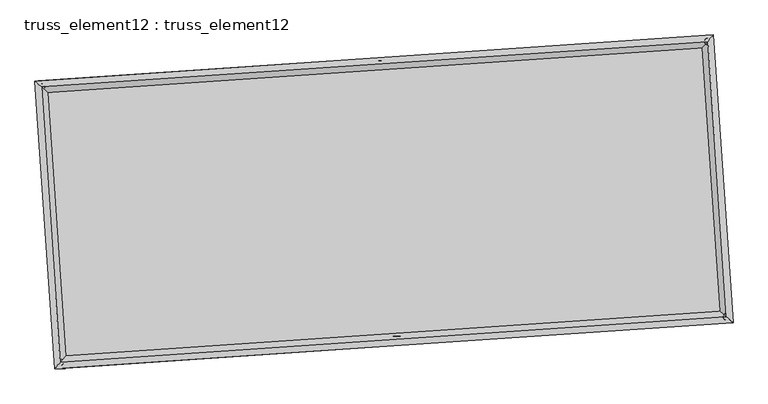
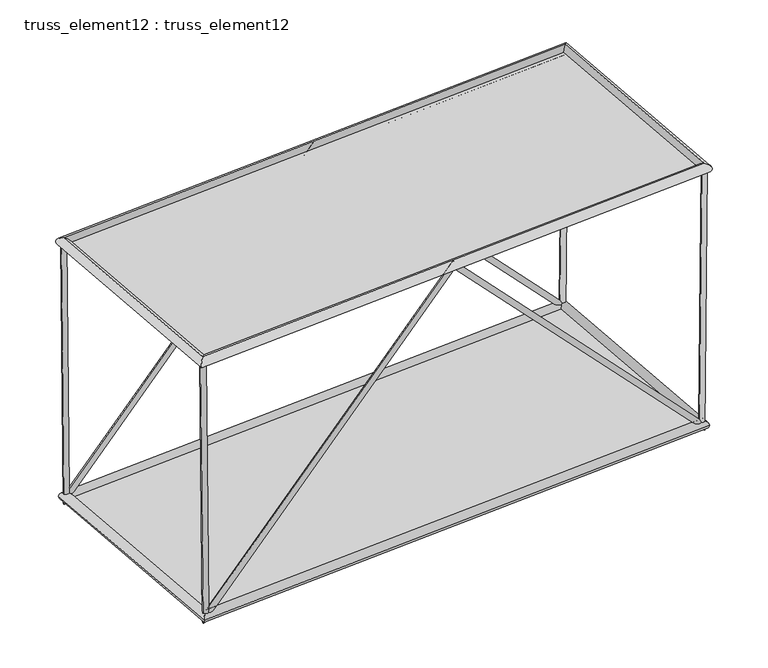
"""IFC4 building model written with IfcOpenShell, lengths in millimetres: plate geometry, truss_element12 : truss_element12."""

import ifcopenshell
import ifcopenshell.guid

model = None  # the IFC model being written
_history = None  # IfcOwnerHistory: only IFC2X3 demands one
_inside = {}  # id of a spatial element -> (the spatial element, [elements in it])
_under = {}  # id of a project, library or spatial element -> (it, [spatial elements below it])
_declared = {}  # id of a project -> (the project, [libraries it declares])
_typed = {}  # id of a type object -> (the type object, [elements of that type])
_made_of = {}  # id of a material, layer set ... -> (it, [elements and type objects made of it])


def new_model(schema):
    """Start an empty IFC model of exactly this schema.

    Asked for "IFC4X3", IfcOpenShell would pick the latest addendum, in which some entities
    have other attributes; the version numbers below select the first issue.
    IFC2X3 requires an IfcOwnerHistory on every rooted entity: one is made here for all.
    """
    global model, _history
    if schema == "IFC4X3":
        model = ifcopenshell.file(schema_version=(4, 3, 0, 0))
    else:
        model = ifcopenshell.file(schema=schema)
    _inside.clear()
    _under.clear()
    _declared.clear()
    _typed.clear()
    _made_of.clear()
    _history = None
    if model.schema == "IFC2X3":
        org = make("IfcOrganization", Name="unknown")
        user = make(
            "IfcPersonAndOrganization",
            ThePerson=make("IfcPerson", FamilyName="unknown"),
            TheOrganization=org,
        )
        app = make(
            "IfcApplication",
            ApplicationDeveloper=org,
            Version="unknown",
            ApplicationFullName="unknown",
            ApplicationIdentifier="unknown",
        )
        _history = make(
            "IfcOwnerHistory",
            OwningUser=user,
            OwningApplication=app,
            ChangeAction="ADDED",
            CreationDate=0,
        )
    return model


def make(cls, **values):
    """One entity of the class cls with the attributes given. An attribute that is None is left unset."""
    return model.create_entity(
        cls, **{name: value for name, value in values.items() if value is not None}
    )


def rooted(cls, **values):
    """An entity with a GlobalId (a new one), such as an element, a storey or a relation."""
    return make(cls, GlobalId=ifcopenshell.guid.new(), OwnerHistory=_history, **values)


def si_unit(unit_type, name, prefix=None):
    """IfcSIUnit, for example si_unit("LENGTHUNIT", "METRE", prefix="MILLI")."""
    return make("IfcSIUnit", UnitType=unit_type, Prefix=prefix, Name=name)


def assignment(units):
    """IfcUnitAssignment: the units of a project."""
    return None if units is None else make("IfcUnitAssignment", Units=units)


def point(xyz):
    """IfcCartesianPoint."""
    return None if xyz is None else make("IfcCartesianPoint", Coordinates=xyz)


def direction(xyz):
    """IfcDirection."""
    return None if xyz is None else make("IfcDirection", DirectionRatios=xyz)


def frame(location, z_axis=None, x_axis=None):
    """IfcAxis2Placement3D, a coordinate frame: its origin and axes. An axis left out is left unset."""
    return make(
        "IfcAxis2Placement3D",
        Location=point(location),
        Axis=direction(z_axis),
        RefDirection=direction(x_axis),
    )


def origin():
    """The frame at (0, 0, 0) with its axes left unset."""
    return frame((0.0, 0.0, 0.0))


def origin_with_axes():
    """The frame at (0, 0, 0) with the z axis (0, 0, 1) and the x axis (1, 0, 0) written out."""
    return frame((0.0, 0.0, 0.0), z_axis=(0.0, 0.0, 1.0), x_axis=(1.0, 0.0, 0.0))


def place(relative_to, where):
    """IfcLocalPlacement: puts the frame where relative to a parent placement (None: the world)."""
    return make(
        "IfcLocalPlacement", PlacementRelTo=relative_to, RelativePlacement=where
    )


def context(
    kind, dimensions, precision=None, world=None, true_north=None, identifier=None
):
    """IfcGeometricRepresentationContext, for example the 3D "Model" context."""
    return make(
        "IfcGeometricRepresentationContext",
        ContextIdentifier=identifier,
        ContextType=kind,
        CoordinateSpaceDimension=dimensions,
        Precision=precision,
        WorldCoordinateSystem=world,
        TrueNorth=true_north,
    )


def project(units=None, contexts=None):
    """IfcProject with its units and contexts."""
    return rooted(
        "IfcProject",
        Name="project",
        RepresentationContexts=contexts,
        UnitsInContext=assignment(units),
    )


def spatial(cls, under=None, at=None, **own):
    """A site, building, storey or space (cls), placed at a placement, below another one or the project."""
    s = rooted(cls, ObjectPlacement=at, **own)
    if under is not None:
        _under.setdefault(under.id(), (under, []))[1].append(s)
    return s


def polyline(points):
    """IfcPolyline through the points."""
    return make("IfcPolyline", Points=[point(p) for p in points])


def circle_curve(where, radius):
    """IfcCircle in the frame where."""
    return make("IfcCircle", Position=where, Radius=radius)


def ellipse_curve(where, semi_axis1, semi_axis2):
    """IfcEllipse in the frame where."""
    return make(
        "IfcEllipse", Position=where, SemiAxis1=semi_axis1, SemiAxis2=semi_axis2
    )


def outline(outer, holes=None, kind="AREA"):
    """IfcArbitraryClosedProfileDef: a profile drawn as a closed curve; with holes, ...WithVoids."""
    if holes is None:
        return make("IfcArbitraryClosedProfileDef", ProfileType=kind, OuterCurve=outer)
    return make(
        "IfcArbitraryProfileDefWithVoids",
        ProfileType=kind,
        OuterCurve=outer,
        InnerCurves=holes,
    )


def extrude(swept, where, along, depth):
    """IfcExtrudedAreaSolid: the profile swept, set in the frame where, extruded along a direction by depth."""
    return make(
        "IfcExtrudedAreaSolid",
        SweptArea=swept,
        Position=where,
        ExtrudedDirection=direction(along),
        Depth=depth,
    )


def shape(context_of_items, identifier, shape_type, items):
    """IfcShapeRepresentation: the items that make up one representation, for example the "Body"."""
    return make(
        "IfcShapeRepresentation",
        ContextOfItems=context_of_items,
        RepresentationIdentifier=identifier,
        RepresentationType=shape_type,
        Items=items,
    )


def source(mapping_origin, context_of_items, identifier, shape_type, items):
    """IfcRepresentationMap: a shape defined once, which mapped items show again and again."""
    return make(
        "IfcRepresentationMap",
        MappingOrigin=mapping_origin,
        MappedRepresentation=shape(context_of_items, identifier, shape_type, items),
    )


def transform(
    local_origin,
    x_axis=None,
    y_axis=None,
    z_axis=None,
    scale=None,
    scale2=None,
    scale3=None,
    uniform=True,
):
    """IfcCartesianTransformationOperator3D, or its non-uniform kind. x_axis, y_axis, z_axis: its Axis1, 2, 3."""
    if uniform:
        return make(
            "IfcCartesianTransformationOperator3D",
            Axis1=direction(x_axis),
            Axis2=direction(y_axis),
            LocalOrigin=point(local_origin),
            Scale=scale,
            Axis3=direction(z_axis),
        )
    return make(
        "IfcCartesianTransformationOperator3DnonUniform",
        Axis1=direction(x_axis),
        Axis2=direction(y_axis),
        LocalOrigin=point(local_origin),
        Scale=scale,
        Axis3=direction(z_axis),
        Scale2=scale2,
        Scale3=scale3,
    )


def mapped(mapping_source, mapping_target):
    """IfcMappedItem: shows the shape of a source again, moved by a transform."""
    return make(
        "IfcMappedItem", MappingSource=mapping_source, MappingTarget=mapping_target
    )


def made_of(thing, what):
    """Note that an element or type object is made of a material, layer set ...; save() writes the relation."""
    if what is not None:
        _made_of.setdefault(what.id(), (what, []))[1].append(thing)
    return thing


def element(
    cls,
    number,
    at=None,
    inside=None,
    cuts=None,
    type_object=None,
    material=None,
    context=None,
    identifier="Body",
    shape_type=None,
    held_by="IfcProductDefinitionShape",
    body=None,
    shapes=None,
    **own,
):
    """One element of the class cls, such as IfcWall. Its Tag is "e" and its number.

    at: its placement. inside: the storey or other place that contains it. cuts: it is an
    opening in that element (IfcRelVoidsElement). A single representation is given by context,
    identifier, shape_type and body (its items); several are given by shapes. held_by: the class
    of the entity that holds the representations. save() writes the other relations.
    """
    e = rooted(cls, Tag="e%d" % number, ObjectPlacement=at, **own)
    if body is not None:
        shapes = [shape(context, identifier, shape_type, body)]
    if shapes is not None:
        e.Representation = make(held_by, Representations=shapes)
    if inside is not None:
        _inside.setdefault(inside.id(), (inside, []))[1].append(e)
    if cuts is not None:
        rooted(
            "IfcRelVoidsElement", RelatingBuildingElement=cuts, RelatedOpeningElement=e
        )
    if type_object is not None:
        _typed.setdefault(type_object.id(), (type_object, []))[1].append(e)
    return made_of(e, material)


def aggregate(whole, parts):
    """IfcRelAggregates: a whole, such as a stair, and the parts it consists of."""
    return rooted("IfcRelAggregates", RelatingObject=whole, RelatedObjects=parts)


def save(model, path):
    """Write the relations noted so far, then the file.

    IfcRelAggregates (storeys below a building ...), IfcRelContainedInSpatialStructure (elements
    in a storey), IfcRelDefinesByType, IfcRelAssociatesMaterial and IfcRelDeclares: one each for
    every whole, place, type object, material and project.
    """
    for whole, parts in _under.values():
        aggregate(whole, parts)
    for where, things in _inside.values():
        rooted(
            "IfcRelContainedInSpatialStructure",
            RelatedElements=things,
            RelatingStructure=where,
        )
    for kind, things in _typed.values():
        rooted("IfcRelDefinesByType", RelatedObjects=things, RelatingType=kind)
    for what, things in _made_of.values():
        rooted("IfcRelAssociatesMaterial", RelatedObjects=things, RelatingMaterial=what)
    for by, libraries in _declared.values():
        rooted("IfcRelDeclares", RelatingContext=by, RelatedDefinitions=libraries)
    model.write(path)


def plane_surface(at):
    """IfcPlane: the flat surface through the origin of the frame at, square to its z axis."""
    return make("IfcPlane", Position=at)


def cylinder_surface(at, radius):
    """IfcCylindricalSurface: all points at the distance radius from the z axis of the frame at."""
    return make("IfcCylindricalSurface", Position=at, Radius=radius)


def advanced_brep(points, edges, surfaces, faces):
    """IfcAdvancedBrep: a solid bounded by faces that lie on surfaces and meet in shared edges.

    An edge is (start, end): straight between two places in points (the first is 0);
    or (start, end, curve); or (start, end, curve, False) where it runs against its curve.
    A face is (place in surfaces, loops), or (place, loops, False) where it looks against
    its surface's normal. A loop lists edges by number (the first is 1), with a minus sign
    where the edge is run from its end to its start. The first loop is the outer one.
    """
    corners = [point(p) for p in points]
    vertices = [make("IfcVertexPoint", VertexGeometry=c) for c in corners]
    made = []
    for start, end, *more in edges:
        made.append(
            make(
                "IfcEdgeCurve",
                EdgeStart=vertices[start],
                EdgeEnd=vertices[end],
                EdgeGeometry=more[0] if more else make("IfcPolyline", Points=[corners[start], corners[end]]),
                SameSense=more[1] if len(more) > 1 else True,
            )
        )
    hull = []
    for where, loops, *sense in faces:
        bounds = []
        for j, loop in enumerate(loops):
            ring = [make("IfcOrientedEdge", EdgeElement=made[abs(k) - 1], Orientation=k > 0) for k in loop]
            bounds.append(
                make(
                    "IfcFaceOuterBound" if j == 0 else "IfcFaceBound",
                    Bound=make("IfcEdgeLoop", EdgeList=ring),
                    Orientation=True,
                )
            )
        hull.append(make("IfcAdvancedFace", Bounds=bounds, FaceSurface=surfaces[where], SameSense=sense[0] if sense else True))
    return make("IfcAdvancedBrep", Outer=make("IfcClosedShell", CfsFaces=hull))


def truss_element12_truss_element12_ac9c6d62(model_context):
    return source(origin(), model_context, "Body", "SolidModel", [
        advanced_brep(
        [(-3716.0930721, 2272.7361645, 5000.2487185), (-3815.1912006, 2259.3752454, 4999.2255971), (-3666.1964298, 2276.1384269, 122.8985351), (-3762.790453, 2262.9482532, -122.8985351), (1063.2705222, 2598.6227999, 5071.8637093), (1063.7254289, 2592.0500239, 4927.6196851), (5793.6135203, 2921.1669073, 122.9048123), (5891.1474567, 2921.2135812, -122.9048123), (5842.6407291, 2924.5098863, 5000.248885), (5942.6354458, 2924.7243515, 4999.2435881)],
        [
            (0, 1, circle_curve(frame((-3765.6421364, 2266.055705, 4999.7371578), z_axis=(-0.010229738989149566, -0.0006975270147916147, 0.9999474315664186), x_axis=(-0.13360930371043286, 0.991033852899563, -0.0006755509311635323)), 50.0)),
            (1, 0, circle_curve(frame((-3765.6421364, 2266.055705, 4999.7371578), z_axis=(-0.010229738989149566, -0.0006975270147916147, 0.9999474315664186), x_axis=(-0.13360930371043286, 0.991033852899563, -0.0006755509311635323)), 50.0)),
            (0, 2),
            (2, 3, ellipse_curve(frame((-3714.4934414, 2269.54334, 0.0), z_axis=(-0.9276876380424472, -0.06325549356725499, 0.36795976513307577), x_axis=(0.367107348096881, 0.02503165456104934, 0.9298417130045371)), 132.4592623, 50.0)),
            (3, 1),
            (3, 2, ellipse_curve(frame((-3714.4934414, 2269.54334, 0.0), z_axis=(-0.9276876380424472, -0.06325549356725499, 0.36795976513307577), x_axis=(0.367107348096881, 0.02503165456104934, 0.9298417130045371)), 132.4592623, 50.0)),
            (2, 4),
            (4, 5, ellipse_curve(frame((1063.4979755, 2595.3364119, 4999.7416972), z_axis=(-0.9976833949926481, -0.0680282381549069, -4.657770887694116e-05), x_axis=(4.6469806773723855e-05, 3.1685994757026087e-06, -0.9999999989152586)), 72.2790583, 50.0)),
            (5, 3),
            (5, 4, ellipse_curve(frame((1063.4979755, 2595.3364119, 4999.7416972), z_axis=(-0.9976833949926481, -0.0680282381549069, -4.657770887694116e-05), x_axis=(4.6469806773723855e-05, 3.1685994757026087e-06, -0.9999999989152586)), 72.2790583, 50.0)),
            (4, 6),
            (6, 7, ellipse_curve(frame((5842.3804885, 2921.1902443, 0.0), z_axis=(-0.9276377400160161, -0.06325209121051292, -0.3680861261382656), x_axis=(-0.3672334163736703, -0.025040250677613285, 0.9297916991157348)), 132.4731533, 50.0)),
            (7, 5),
            (7, 6, ellipse_curve(frame((5842.3804885, 2921.1902443, 0.0), z_axis=(-0.9276377400160161, -0.06325209121051292, -0.3680861261382656), x_axis=(-0.3672334163736703, -0.025040250677613285, 0.9297916991157348)), 132.4731533, 50.0)),
            (8, 9, circle_curve(frame((5892.6380875, 2924.6171189, 4999.7462366), z_axis=(0.010051519791738127, 0.000685374925194703, 0.9999492473176268), x_axis=(-0.0021514333546637375, 0.9999974653609742, -0.0006637817017735374)), 50.0)),
            (9, 8, circle_curve(frame((5892.6380875, 2924.6171189, 4999.7462366), z_axis=(0.010051519791738127, 0.000685374925194703, 0.9999492473176268), x_axis=(-0.0021514333546637375, 0.9999974653609742, -0.0006637817017735374)), 50.0)),
            (6, 8),
            (9, 7),
        ],
        [
            plane_surface(frame((-3765.6421364, 2316.0556928, 4999.772036), z_axis=(-0.01022973898914786, -0.0006975270147901555, 0.9999474315664189), x_axis=(0.9999476748511464, -7.13589268563908e-06, 0.010229736500278365))),
            cylinder_surface(frame((-3765.6421364, 2266.055705, 4999.7371578), z_axis=(-0.010229738989149566, -0.0006975270147916147, 0.9999474315664186), x_axis=(-0.13360930371043286, 0.991033852899563, -0.0006755509311635323)), 50.0),
            cylinder_surface(frame((-3714.4934414, 2269.54334, 0.0), z_axis=(-0.6901272026448979, -0.047057150529254535, -0.722156540338447), x_axis=(-0.02041139550442059, 0.9987523879545969, -0.04557458160589792)), 50.0),
            cylinder_surface(frame((1063.4979755, 2595.3364119, 4999.7416972), z_axis=(-0.6901943166001666, -0.047061726774740395, 0.7220920988390669), x_axis=(-0.11534522502427148, 0.9922792109969094, -0.04557901367352192)), 50.0),
            plane_surface(frame((5892.6380875, 2874.6171306, 4999.7805071), z_axis=(0.010051519791740156, 0.0006853749251952957, 0.9999492473176268), x_axis=(0.9999494821989141, -6.889407663024368e-06, -0.010051517430706975))),
            cylinder_surface(frame((5842.3804885, 2921.1902443, 0.0), z_axis=(-0.010051519791738127, -0.000685374925194703, -0.9999492473176268), x_axis=(-0.0021514333546637375, 0.9999974653609742, -0.0006637817017735374)), 50.0),
        ],
        [
            (0, [[1, 2]]),
            (1, [[-1, 3, 4, 5]]),
            (1, [[-2, -5, 6, -3]]),
            (2, [[-4, 7, 8, 9]]),
            (2, [[-6, -9, 10, -7]]),
            (3, [[-8, 11, 12, 13]]),
            (3, [[-10, -13, 14, -11]]),
            (4, [[15, 16]]),
            (5, [[-12, 17, -16, 18]]),
            (5, [[-14, -18, -15, -17]]),
        ],
    ),
        advanced_brep(
        [(-3443.9801192, -1717.9974198, 5000.2487185), (-3543.0782477, -1731.3583389, 4999.2255971), (-3394.0834769, -1714.5951574, 122.8985351), (-3490.6775001, -1727.7853311, -122.8985351), (1335.3834751, -1392.1107844, 5071.8637093), (1335.8383818, -1398.6835604, 4927.6196851), (6065.7264732, -1069.566677, 122.9048123), (6163.2604096, -1069.5200031, -122.9048123), (6114.753682, -1066.223698, 5000.248885), (6214.7483988, -1066.0092328, 4999.2435881)],
        [
            (0, 1, circle_curve(frame((-3493.5291834, -1724.6778793, 4999.7371578), z_axis=(-0.010229738989149568, -0.0006975270147916012, 0.9999474315664186), x_axis=(-0.1336093037104329, 0.991033852899563, -0.0006755509311635461)), 50.0)),
            (1, 0, circle_curve(frame((-3493.5291834, -1724.6778793, 4999.7371578), z_axis=(-0.010229738989149568, -0.0006975270147916012, 0.9999474315664186), x_axis=(-0.1336093037104329, 0.991033852899563, -0.0006755509311635461)), 50.0)),
            (0, 2),
            (2, 3, ellipse_curve(frame((-3442.3804885, -1721.1902443, 0.0), z_axis=(-0.9276876380424474, -0.06325549356725498, 0.3679597651330757), x_axis=(0.3671073480968811, 0.025031654561049346, 0.9298417130045371)), 132.4592623, 50.0)),
            (3, 1),
            (3, 2, ellipse_curve(frame((-3442.3804885, -1721.1902443, 0.0), z_axis=(-0.9276876380424474, -0.06325549356725498, 0.3679597651330757), x_axis=(0.3671073480968811, 0.025031654561049346, 0.9298417130045371)), 132.4592623, 50.0)),
            (2, 4),
            (4, 5, ellipse_curve(frame((1335.6109285, -1395.3971724, 4999.7416972), z_axis=(-0.9976833949926481, -0.06802823815490679, -4.657770887694117e-05), x_axis=(4.6469806773723855e-05, 3.1685994756065187e-06, -0.9999999989152586)), 72.2790583, 50.0)),
            (5, 3),
            (5, 4, ellipse_curve(frame((1335.6109285, -1395.3971724, 4999.7416972), z_axis=(-0.9976833949926481, -0.06802823815490679, -4.657770887694117e-05), x_axis=(4.6469806773723855e-05, 3.1685994756065187e-06, -0.9999999989152586)), 72.2790583, 50.0)),
            (4, 6),
            (6, 7, ellipse_curve(frame((6114.4934414, -1069.54334, 0.0), z_axis=(-0.9276377400160161, -0.0632520912105128, -0.3680861261382654), x_axis=(-0.3672334163736703, -0.02504025067761318, 0.9297916991157348)), 132.4731533, 50.0)),
            (7, 5),
            (7, 6, ellipse_curve(frame((6114.4934414, -1069.54334, 0.0), z_axis=(-0.9276377400160161, -0.0632520912105128, -0.3680861261382654), x_axis=(-0.3672334163736703, -0.02504025067761318, 0.9297916991157348)), 132.4731533, 50.0)),
            (8, 9, circle_curve(frame((6164.7510404, -1066.1164654, 4999.7462366), z_axis=(0.010051519791738519, 0.0006853749251947742, 0.9999492473176269), x_axis=(-0.0021514333546638212, 0.9999974653609742, -0.0006637817017736069)), 50.0)),
            (9, 8, circle_curve(frame((6164.7510404, -1066.1164654, 4999.7462366), z_axis=(0.010051519791738519, 0.0006853749251947742, 0.9999492473176269), x_axis=(-0.0021514333546638212, 0.9999974653609742, -0.0006637817017736069)), 50.0)),
            (6, 8),
            (9, 7),
        ],
        [
            plane_surface(frame((-3493.5291834, -1674.6778915, 4999.772036), z_axis=(-0.01022973898914786, -0.0006975270147901575, 0.9999474315664189), x_axis=(0.9999476748511464, -7.13589268563908e-06, 0.010229736500278365))),
            cylinder_surface(frame((-3493.5291834, -1724.6778793, 4999.7371578), z_axis=(-0.010229738989149568, -0.0006975270147916012, 0.9999474315664186), x_axis=(-0.1336093037104329, 0.991033852899563, -0.0006755509311635461)), 50.0),
            cylinder_surface(frame((-3442.3804885, -1721.1902443, 0.0), z_axis=(-0.6901272026448979, -0.04705715052925453, -0.7221565403384471), x_axis=(-0.02041139550442058, 0.9987523879545969, -0.04557458160589791)), 50.0),
            cylinder_surface(frame((1335.6109285, -1395.3971724, 4999.7416972), z_axis=(-0.6901943166001666, -0.047061726774740256, 0.7220920988390671), x_axis=(-0.11534522502427137, 0.9922792109969095, -0.04557901367352197)), 50.0),
            plane_surface(frame((6164.7510404, -1116.1164537, 4999.7805071), z_axis=(0.010051519791740156, 0.0006853749251952975, 0.9999492473176268), x_axis=(0.9999494821989141, -6.889407663024368e-06, -0.010051517430706975))),
            cylinder_surface(frame((6114.4934414, -1069.54334, 0.0), z_axis=(-0.010051519791738517, -0.0006853749251947741, -0.9999492473176267), x_axis=(-0.0021514333546638212, 0.9999974653609742, -0.0006637817017736069)), 50.0),
        ],
        [
            (0, [[1, 2]]),
            (1, [[-1, 3, 4, 5]]),
            (1, [[-2, -5, 6, -3]]),
            (2, [[-4, 7, 8, 9]]),
            (2, [[-6, -9, 10, -7]]),
            (3, [[-8, 11, 12, 13]]),
            (3, [[-10, -13, 14, -11]]),
            (4, [[15, 16]]),
            (5, [[-12, 17, -16, 18]]),
            (5, [[-14, -18, -15, -17]]),
        ],
    ),
        advanced_brep(
        [(-3493.526795, -1724.6752322, 4909.7371579), (-3493.5315719, -1724.6805265, 5089.7371578), (-3765.644862, 2266.0580034, 5089.7371578), (-3765.6394107, 2266.0534065, 4909.7371579), (5892.6403075, 2924.6197546, 5089.7462366), (5892.6358675, 2924.6144832, 4909.7462366), (6164.7535976, -1066.1187754, 5089.7462366), (6164.7484832, -1066.1141555, 4909.7462366)],
        [
            (0, 1, ellipse_curve(frame((-3493.5291834, -1724.6778793, 4999.7371578), z_axis=(-0.7535719234051438, 0.6573654662781065, -6.631385733945912e-07), x_axis=(-0.6573654662777754, -0.7535719234054328, -6.631385733946736e-07)), 127.2792206, 90.0)),
            (1, 2),
            (2, 3, ellipse_curve(frame((-3765.6421364, 2266.055705, 4999.7371578), z_axis=(-0.6573654662777749, -0.753571923405433, -6.631385733947504e-07), x_axis=(0.753571923405144, -0.6573654662781062, 6.631385733946685e-07)), 127.2792206, 90.0)),
            (3, 0),
            (1, 0, ellipse_curve(frame((-3493.5291834, -1724.6778793, 4999.7371578), z_axis=(-0.7535719234051438, 0.6573654662781065, -6.631385733945912e-07), x_axis=(-0.6573654662777754, -0.7535719234054328, -6.631385733946736e-07)), 127.2792206, 90.0)),
            (3, 2, ellipse_curve(frame((-3765.6421364, 2266.055705, 4999.7371578), z_axis=(-0.6573654662777749, -0.753571923405433, -6.631385733947504e-07), x_axis=(0.753571923405144, -0.6573654662781062, 6.631385733946685e-07)), 127.2792206, 90.0)),
            (2, 4),
            (4, 5, ellipse_curve(frame((5892.6380875, 2924.6171189, 4999.7462366), z_axis=(-0.7535719234051438, 0.6573654662781065, -6.631385733947457e-07), x_axis=(-0.657365466277775, -0.7535719234054329, -6.63138573394673e-07)), 127.2792206, 90.0)),
            (5, 3),
            (5, 4, ellipse_curve(frame((5892.6380875, 2924.6171189, 4999.7462366), z_axis=(-0.7535719234051438, 0.6573654662781065, -6.631385733947457e-07), x_axis=(-0.657365466277775, -0.7535719234054329, -6.63138573394673e-07)), 127.2792206, 90.0)),
            (4, 6),
            (6, 7, ellipse_curve(frame((6164.7510404, -1066.1164654, 4999.7462366), z_axis=(0.6573654662777753, 0.7535719234054328, 6.631385733945962e-07), x_axis=(-0.7535719234051438, 0.6573654662781064, -6.631385733946685e-07)), 127.2792206, 90.0)),
            (7, 5),
            (7, 6, ellipse_curve(frame((6164.7510404, -1066.1164654, 4999.7462366), z_axis=(0.6573654662777753, 0.7535719234054328, 6.631385733945962e-07), x_axis=(-0.7535719234051438, 0.6573654662781064, -6.631385733946685e-07)), 127.2792206, 90.0)),
            (6, 1),
            (0, 7),
        ],
        [
            cylinder_surface(frame((-3493.5291834, -1724.6778793, 4999.7371578), z_axis=(0.06802823822869494, -0.997683396074877, 0.0), x_axis=(-0.9976833956703363, -0.06802823820111085, -2.8477362265498946e-05)), 90.0),
            cylinder_surface(frame((-3765.6421364, 2266.055705, 4999.7371578), z_axis=(-0.9976833960744383, -0.06802823822866604, -9.378195642275444e-07), x_axis=(-0.06802823817713145, 0.9976833956982993, -2.7539542701627088e-05)), 90.0),
            cylinder_surface(frame((5892.6380875, 2924.6171189, 4999.7462366), z_axis=(-0.06802823822869457, 0.9976833960748772, 0.0), x_axis=(0.997683395721871, 0.06802823820462442, -2.6601723137755227e-05)), 90.0),
            cylinder_surface(frame((6164.7510404, -1066.1164654, 4999.7462366), z_axis=(0.9976833960744383, 0.06802823822866567, 9.378195642274352e-07), x_axis=(0.06802823822866567, -0.9976833956947854, -2.753954270162708e-05)), 90.0),
        ],
        [
            (0, [[1, 2, 3, 4]]),
            (0, [[5, -4, 6, -2]]),
            (1, [[-3, 7, 8, 9]]),
            (1, [[-6, -9, 10, -7]]),
            (2, [[-8, 11, 12, 13]]),
            (2, [[-10, -13, 14, -11]]),
            (3, [[-12, 15, -1, 16]]),
            (3, [[-14, -16, -5, -15]]),
        ],
    ),
        advanced_brep(
        [(-3358.7115243, -1625.2761972, 0.0), (-3526.0494527, -1817.1042913, 0.0), (-3810.4074885, 2353.2123043, 0.0), (-3618.5793943, 2185.8743758, 0.0), (5926.0494527, 3017.1042913, 0.0), (5758.7115243, 2825.2761972, 0.0), (6210.4074885, -1153.2123043, 0.0), (6018.5793943, -985.8743758, 0.0)],
        [
            (0, 1, ellipse_curve(frame((-3442.3804885, -1721.1902443, 0.0), z_axis=(-0.7535719234054566, 0.6573654662780822, 0.0), x_axis=(-0.6573654662780821, -0.7535719234054568, 0.0)), 127.2792206, 90.0)),
            (1, 2),
            (2, 3, ellipse_curve(frame((-3714.4934414, 2269.54334, 0.0), z_axis=(-0.6573654662780822, -0.7535719234054568, 0.0), x_axis=(0.7535719234054568, -0.6573654662780821, 0.0)), 127.2792206, 90.0)),
            (3, 0),
            (1, 0, ellipse_curve(frame((-3442.3804885, -1721.1902443, 0.0), z_axis=(-0.7535719234054566, 0.6573654662780822, 0.0), x_axis=(-0.6573654662780821, -0.7535719234054568, 0.0)), 127.2792206, 90.0)),
            (3, 2, ellipse_curve(frame((-3714.4934414, 2269.54334, 0.0), z_axis=(-0.6573654662780822, -0.7535719234054568, 0.0), x_axis=(0.7535719234054568, -0.6573654662780821, 0.0)), 127.2792206, 90.0)),
            (2, 4),
            (4, 5, ellipse_curve(frame((5842.3804885, 2921.1902443, 0.0), z_axis=(-0.7535719234054566, 0.6573654662780823, 0.0), x_axis=(-0.6573654662780822, -0.7535719234054566, 0.0)), 127.2792206, 90.0)),
            (5, 3),
            (5, 4, ellipse_curve(frame((5842.3804885, 2921.1902443, 0.0), z_axis=(-0.7535719234054566, 0.6573654662780823, 0.0), x_axis=(-0.6573654662780822, -0.7535719234054566, 0.0)), 127.2792206, 90.0)),
            (4, 6),
            (6, 7, ellipse_curve(frame((6114.4934414, -1069.54334, 0.0), z_axis=(0.6573654662780825, 0.7535719234054565, 0.0), x_axis=(-0.7535719234054565, 0.6573654662780825, 0.0)), 127.2792206, 90.0)),
            (7, 5),
            (7, 6, ellipse_curve(frame((6114.4934414, -1069.54334, 0.0), z_axis=(0.6573654662780825, 0.7535719234054565, 0.0), x_axis=(-0.7535719234054565, 0.6573654662780825, 0.0)), 127.2792206, 90.0)),
            (6, 1),
            (0, 7),
        ],
        [
            cylinder_surface(frame((-3442.3804885, -1721.1902443, 0.0), z_axis=(0.06802823822869897, -0.9976833960748768, 0.0), x_axis=(-0.9976833960748768, -0.06802823822869897, 0.0)), 90.0),
            cylinder_surface(frame((-3714.4934414, 2269.54334, 0.0), z_axis=(-0.9976833960748768, -0.06802823822869992, 0.0), x_axis=(-0.06802823822869992, 0.9976833960748768, 0.0)), 90.0),
            cylinder_surface(frame((5842.3804885, 2921.1902443, 0.0), z_axis=(-0.06802823822869855, 0.9976833960748768, 0.0), x_axis=(0.9976833960748768, 0.06802823822869855, 0.0)), 90.0),
            cylinder_surface(frame((6114.4934414, -1069.54334, 0.0), z_axis=(0.9976833960748768, 0.06802823822869959, 0.0), x_axis=(0.06802823822869959, -0.9976833960748768, 0.0)), 90.0),
        ],
        [
            (0, [[1, 2, 3, 4]]),
            (0, [[5, -4, 6, -2]]),
            (1, [[-3, 7, 8, 9]]),
            (1, [[-6, -9, 10, -7]]),
            (2, [[-8, 11, 12, 13]]),
            (2, [[-10, -13, 14, -11]]),
            (3, [[-12, 15, -1, 16]]),
            (3, [[-14, -16, -5, -15]]),
        ],
    ),
        extrude(outline(polyline([(-3442.3804885, -1721.1902443), (-3714.4934414, 2269.54334), (5842.3804885, 2921.1902443), (6114.4934414, -1069.54334), (-3442.3804885, -1721.1902443)])), origin_with_axes(), (0.0, 0.0, 1.0), 20.0),
        extrude(outline(polyline([(-2000.0, 4840.3532933), (2000.0, 4840.3532934), (2000.0, -4840.3532934), (-2000.0, -4840.3532934), (-2000.0, 4840.3532933)])), frame((1199.554452, 599.9696198, 4999.7416972), z_axis=(-9.356470077439426e-07, -6.379821273080194e-08, 0.9999999999995604), x_axis=(-0.06802823822869858, 0.9976833960748768, 0.0)), (0.0, 0.0, 1.0), 20.0),
    ])


if __name__ == "__main__":
    model = new_model("IFC4")
    model_context = context("Model", 3, world=origin())
    ifc_project = project(units=[si_unit("LENGTHUNIT", "METRE", prefix="MILLI")], contexts=[model_context])
    site = spatial("IfcSite", under=ifc_project)
    building = spatial("IfcBuilding", under=site)
    placement = place(None, origin())
    truss_element12_truss_element12_shape = truss_element12_truss_element12_ac9c6d62(model_context)
    element("IfcPlate", 1, ObjectType="truss_element12 : truss_element12", at=placement, inside=building, context=model_context, shape_type="MappedRepresentation", body=[
        mapped(truss_element12_truss_element12_shape, transform((0.0, 0.0, 0.0), x_axis=(1.0, 0.0, 0.0), y_axis=(0.0, 1.0, 0.0), z_axis=(0.0, 0.0, 1.0))),
    ])
    save(model, "model.ifc")

# Revit data of these elements
# Type "truss_element12 : truss_element12"
#   steellbar1 = 90 mm
#   steelbar2 = 50 mm
#   offset1 = 5000 mm
#   M = Default Roof
# Element 1 (IfcPlate, "truss_element12 : truss_element12")
#   Materials on its faces: "Default Roof"
# Materials
#   "Default Roof": class "Miscellaneous", colour RGB 0 127 0, transparency 0, Comments = "Rendering appearance not upgraded Rendering appearance not upgraded ", Cost = 0
